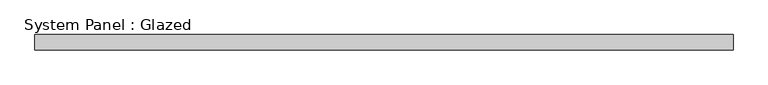
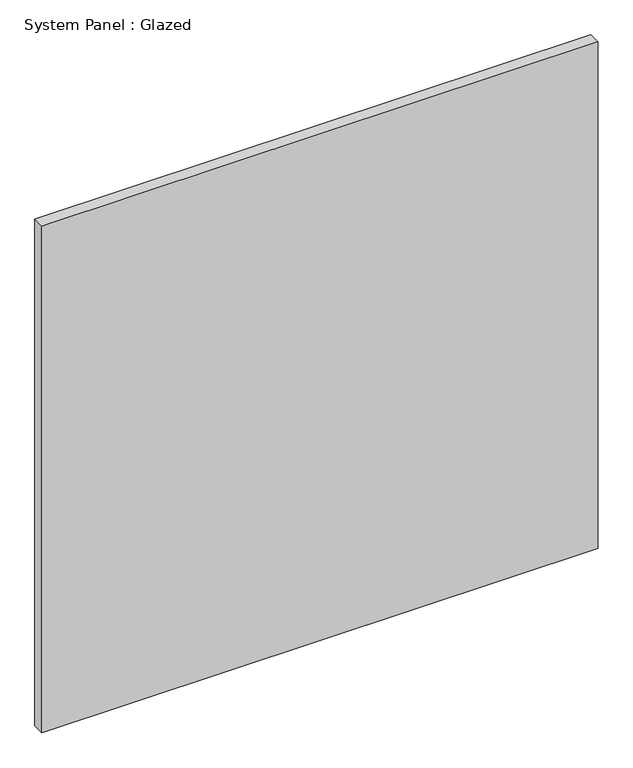
"""IFC4 building model written with IfcOpenShell, lengths in millimetres: plate geometry, System Panel : Glazed."""

from ifc_helpers import new_model, si_unit, origin, origin_with_axes, place, context, project, spatial, polyline, outline, extrude, source, transform, mapped, element, save


def system_panel_glazed_81eeab3d(model_context):
    return source(origin(), model_context, "Body", "SweptSolid", [
        extrude(outline(polyline([(583.1416667, 19.05), (-583.1416667, 19.05), (-583.1416667, 44.45), (583.1416667, 44.45), (583.1416667, 19.05)])), origin_with_axes(), (0.0, 0.0, 1.0), 1123.95),
    ])


if __name__ == "__main__":
    model = new_model("IFC4")
    model_context = context("Model", 3, world=origin())
    ifc_project = project(units=[si_unit("LENGTHUNIT", "METRE", prefix="MILLI")], contexts=[model_context])
    site = spatial("IfcSite", under=ifc_project)
    building = spatial("IfcBuilding", under=site)
    placement = place(None, origin())
    system_panel_glazed_shape = system_panel_glazed_81eeab3d(model_context)
    element("IfcPlate", 1, ObjectType="System Panel : Glazed", at=placement, inside=building, context=model_context, shape_type="MappedRepresentation", body=[
        mapped(system_panel_glazed_shape, transform((0.0, 0.0, 0.0), x_axis=(1.0, 0.0, 0.0), y_axis=(0.0, 1.0, 0.0), z_axis=(0.0, 0.0, 1.0))),
    ])
    save(model, "model.ifc")

# Revit data of these elements
# Element 1 (IfcPlate, "System Panel : Glazed")
#   Materials on its faces: "Glass"
# Materials
#   "Glass": class "Glass", colour RGB 218 227 224, transparency 0.85, Description = "Soda Lime Glass", Cost = 0
